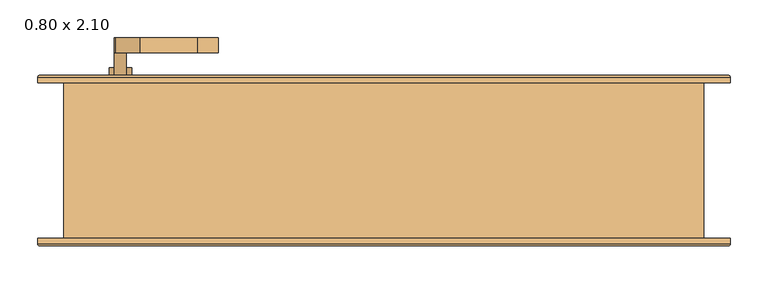
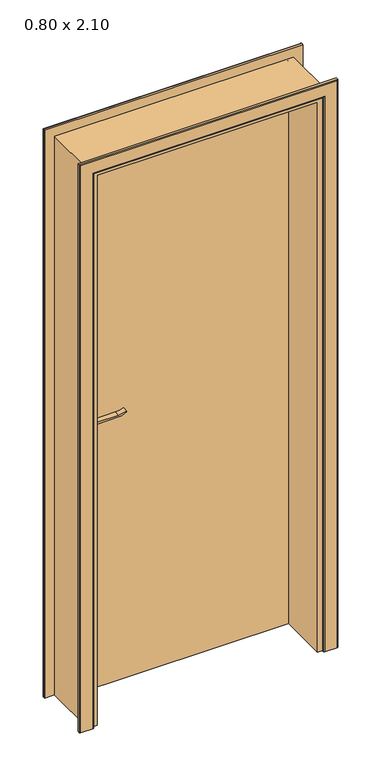
"""IFC4 building model written with IfcOpenShell, lengths in millimetres: door geometry, .CC_ND 300_PORTA SIMPLES DE ABRIR_COM EXTENSÃO : 0.80 x 2.10."""

from ifc_helpers import new_model, si_unit, point, frame, frame_2d, origin, origin_with_axes, place, context, project, spatial, polyline, circle_curve, ellipse_curve, trimmed, segment, composite_curve, outline, extrude, faceted_brep, source, transform, mapped, element, save
from ifc_brep_helpers import plane_surface, cylinder_surface, advanced_brep


def door_0_80_x_2_10_30072744(model_context):
    return source(origin(), model_context, "Body", "SolidModel", [
        extrude(outline(composite_curve([segment(trimmed(circle_curve(frame_2d((964.5, -350.0)), 15.0), [point((964.5, -335.0))], [point((964.5, -365.0))], False, "CARTESIAN"), True, "CONTINUOUS"), segment(trimmed(circle_curve(frame_2d((964.5, -350.0)), 15.0), [point((964.5, -365.0))], [point((964.5, -335.0))], False, "CARTESIAN"), True, "CONTINUOUS")], self_intersect=False)), frame((0.0, 110.7, 0.0), z_axis=(0.0, 1.0, 0.0), x_axis=(0.0, 0.0, 1.0)), (0.0, 0.0, 1.0), 10.0),
        extrude(outline(composite_curve([segment(trimmed(circle_curve(frame_2d((964.5, -350.0)), 15.0), [point((964.5, -335.0))], [point((964.5, -365.0))], False, "CARTESIAN"), True, "CONTINUOUS"), segment(trimmed(circle_curve(frame_2d((964.5, -350.0)), 15.0), [point((964.5, -365.0))], [point((964.5, -335.0))], False, "CARTESIAN"), True, "CONTINUOUS")], self_intersect=False)), frame((0.0, 50.7, 0.0), z_axis=(0.0, 1.0, 0.0), x_axis=(0.0, 0.0, 1.0)), (0.0, 0.0, 1.0), 10.0),
        extrude(outline(composite_curve([segment(trimmed(circle_curve(frame_2d((1024.5, -350.0)), 8.0), [point((1029.1523287, -356.5081363))], [point((1024.5, -342.0))], False, "CARTESIAN"), True, "CONTINUOUS"), segment(trimmed(circle_curve(frame_2d((1019.3738613, -324.6138099)), 18.1261387), [point((1024.5, -342.0))], [point((1037.5, -324.6138099))], True, "CARTESIAN"), True, "CONTINUOUS"), segment(polyline([(1037.5, -324.6138099), (1037.5, -248.3564091)]), True, "CONTINUOUS"), segment(trimmed(circle_curve(frame_2d((1096.7709207, -251.9396612)), 59.3791355), [point((1037.5, -248.3564091))], [point((1046.7135558, -220.0))], False, "CARTESIAN"), True, "CONTINUOUS"), segment(polyline([(1046.7135558, -220.0), (1049.5, -220.0)]), True, "CONTINUOUS"), segment(trimmed(circle_curve(frame_2d((1127.7850638, -248.4227909)), 83.2850902), [point((1049.5, -220.0))], [point((1044.5, -248.3564091))], True, "CARTESIAN"), True, "CONTINUOUS"), segment(polyline([(1044.5, -248.3564091), (1044.5, -324.6325667)]), True, "CONTINUOUS"), segment(trimmed(circle_curve(frame_2d((1007.2555521, -326.3324871)), 37.2832219), [point((1044.5, -324.6325667))], [point((1029.1523287, -356.5081363))], False, "CARTESIAN"), True, "CONTINUOUS")], self_intersect=False)), frame((0.0, 140.7, 0.0), z_axis=(0.0, 1.0, 0.0), x_axis=(0.0, 0.0, 1.0)), (0.0, 0.0, 1.0), 20.0),
        extrude(outline(composite_curve([segment(trimmed(circle_curve(frame_2d((1019.3738682, -324.6138122)), 18.1261318), [point((1024.4999903, -342.0))], [point((1037.5, -324.6138122))], True, "CARTESIAN"), True, "CONTINUOUS"), segment(polyline([(1037.5, -324.6138122), (1037.5, -248.3564091)]), True, "CONTINUOUS"), segment(trimmed(circle_curve(frame_2d((1096.7709207, -251.9396612)), 59.3791355), [point((1037.5, -248.3564091))], [point((1046.7135558, -220.0))], False, "CARTESIAN"), True, "CONTINUOUS"), segment(polyline([(1046.7135558, -220.0), (1049.5, -220.0)]), True, "CONTINUOUS"), segment(trimmed(circle_curve(frame_2d((1127.7850638, -248.4227909)), 83.2850902), [point((1049.5, -220.0))], [point((1044.5, -248.3564091))], True, "CARTESIAN"), True, "CONTINUOUS"), segment(polyline([(1044.5, -248.3564091), (1044.5, -324.6325667)]), True, "CONTINUOUS"), segment(trimmed(circle_curve(frame_2d((1007.2555521, -326.3324871)), 37.2832219), [point((1044.5, -324.6325667))], [point((1029.1523287, -356.5081363))], False, "CARTESIAN"), True, "CONTINUOUS"), segment(trimmed(circle_curve(frame_2d((1024.5, -350.0)), 8.0), [point((1029.1523287, -356.5081363))], [point((1024.4999903, -342.0))], False, "CARTESIAN"), True, "CONTINUOUS")], self_intersect=False)), frame((0.0, 10.7, 0.0), z_axis=(0.0, 1.0, 0.0), x_axis=(0.0, 0.0, 1.0)), (0.0, 0.0, 1.0), 20.0),
        extrude(outline(composite_curve([segment(trimmed(circle_curve(frame_2d((1024.5, -350.0)), 8.0), [point((1024.5, -342.0))], [point((1024.5, -358.0))], False, "CARTESIAN"), True, "CONTINUOUS"), segment(trimmed(circle_curve(frame_2d((1024.5, -350.0)), 8.0), [point((1024.5, -358.0))], [point((1024.5, -342.0))], False, "CARTESIAN"), True, "CONTINUOUS")], self_intersect=False)), frame((0.0, 110.7, 0.0), z_axis=(0.0, 1.0, 0.0), x_axis=(0.0, 0.0, 1.0)), (0.0, 0.0, 1.0), 30.0),
        extrude(outline(composite_curve([segment(trimmed(circle_curve(frame_2d((1024.5, -350.0)), 8.0), [point((1024.5, -342.0))], [point((1024.5, -358.0))], False, "CARTESIAN"), True, "CONTINUOUS"), segment(trimmed(circle_curve(frame_2d((1024.5, -350.0)), 8.0), [point((1024.5, -358.0))], [point((1024.5, -342.0))], False, "CARTESIAN"), True, "CONTINUOUS")], self_intersect=False)), frame((0.0, 30.7, 0.0), z_axis=(0.0, 1.0, 0.0), x_axis=(0.0, 0.0, 1.0)), (0.0, 0.0, 1.0), 30.0),
        extrude(outline(composite_curve([segment(trimmed(circle_curve(frame_2d((954.5, -350.0)), 25.0), [point((954.5, -375.0))], [point((954.5, -325.0))], False, "CARTESIAN"), True, "CONTINUOUS"), segment(polyline([(954.5, -325.0), (1024.5, -325.0)]), True, "CONTINUOUS"), segment(trimmed(circle_curve(frame_2d((1024.5, -350.0)), 25.0), [point((1024.5, -325.0))], [point((1024.5, -375.0))], False, "CARTESIAN"), True, "CONTINUOUS"), segment(polyline([(1024.5, -375.0), (954.5, -375.0)]), True, "CONTINUOUS")], self_intersect=False)), frame((0.0, 100.7, 0.0), z_axis=(0.0, 1.0, 0.0), x_axis=(0.0, 0.0, 1.0)), (0.0, 0.0, 1.0), 10.0),
        extrude(outline(composite_curve([segment(trimmed(circle_curve(frame_2d((954.5, -350.0)), 25.0), [point((954.5, -375.0))], [point((954.5, -325.0))], False, "CARTESIAN"), True, "CONTINUOUS"), segment(polyline([(954.5, -325.0), (1024.5, -325.0)]), True, "CONTINUOUS"), segment(trimmed(circle_curve(frame_2d((1024.5, -350.0)), 25.0), [point((1024.5, -325.0))], [point((1024.5, -375.0))], False, "CARTESIAN"), True, "CONTINUOUS"), segment(polyline([(1024.5, -375.0), (954.5, -375.0)]), True, "CONTINUOUS")], self_intersect=False)), frame((0.0, 60.7, 0.0), z_axis=(0.0, 1.0, 0.0), x_axis=(0.0, 0.0, 1.0)), (0.0, 0.0, 1.0), 10.0),
        faceted_brep([(392.0, -106.0, 0.0), (392.0, 70.7, 0.0), (400.0, 70.7, 0.0), (400.0, 100.7, 0.0), (425.0, 100.7, 0.0), (425.0, -106.0, 0.0), (425.0, -106.0, 2100.0), (-425.0, -106.0, 2100.0), (-425.0, -106.0, 0.0), (-392.0, -106.0, 0.0), (-392.0, -106.0, 2067.0), (392.0, -106.0, 2067.0), (425.0, 100.7, 2100.0), (400.0, 100.7, 2075.0), (-400.0, 100.7, 2075.0), (-400.0, 100.7, 0.0), (-425.0, 100.7, 0.0), (-425.0, 100.7, 2100.0), (400.0, 70.7, 2075.0), (392.0, 70.7, 2067.0), (-392.0, 70.7, 2067.0), (-392.0, 70.7, 0.0), (-400.0, 70.7, 0.0), (-400.0, 70.7, 2075.0)], [[[0, 1, 2, 3, 4, 5]], [[5, 6, 7, 8, 9, 10, 11, 0]], [[4, 12, 6, 5]], [[3, 13, 14, 15, 16, 17, 12, 4]], [[2, 18, 13, 3]], [[1, 19, 20, 21, 22, 23, 18, 2]], [[0, 11, 19, 1]], [[10, 9, 21, 20]], [[9, 8, 16, 15, 22, 21]], [[17, 16, 8, 7]], [[23, 22, 15, 14]], [[12, 17, 7, 6]], [[18, 23, 14, 13]], [[11, 10, 20, 19]]]),
        extrude(outline(polyline([(-400.0, 70.7), (-400.0, 100.7), (400.0, 100.7), (400.0, 70.7), (-400.0, 70.7)])), origin_with_axes(), (0.0, 0.0, 1.0), 2075.0),
        advanced_brep(
        [(-460.0, 100.7, 0.0), (-460.0, 107.7, 0.0), (-457.0, 110.7, 0.0), (-413.0, 110.7, 0.0), (-410.0, 107.7, 0.0), (-410.0, 100.7, 0.0), (-410.0, 100.7, 2085.0), (410.0, 100.7, 2085.0), (410.0, 100.7, 0.0), (460.0, 100.7, 0.0), (460.0, 100.7, 2135.0), (-460.0, 100.7, 2135.0), (-410.0, 107.7, 2085.0), (-413.0, 110.7, 2088.0), (-457.0, 110.7, 2132.0), (457.0, 110.7, 2132.0), (457.0, 110.7, 0.0), (413.0, 110.7, 0.0), (413.0, 110.7, 2088.0), (-460.0, 107.7, 2135.0), (460.0, 107.7, 0.0), (460.0, 107.7, 2135.0), (410.0, 107.7, 0.0), (410.0, 107.7, 2085.0)],
        [
            (0, 1),
            (1, 2, circle_curve(frame((-457.0, 107.7, 0.0), z_axis=(0.0, 0.0, -1.0), x_axis=(1.0, 0.0, 0.0)), 3.0)),
            (2, 3),
            (3, 4, circle_curve(frame((-413.0, 107.7, 0.0), z_axis=(0.0, 0.0, -1.0), x_axis=(1.0, 0.0, 0.0)), 3.0)),
            (4, 5),
            (5, 0),
            (5, 6),
            (6, 7),
            (7, 8),
            (8, 9),
            (9, 10),
            (10, 11),
            (11, 0),
            (4, 12),
            (12, 6),
            (3, 13),
            (13, 12, ellipse_curve(frame((-413.0, 107.7, 2088.0), z_axis=(-0.7071067811865475, 0.0, -0.7071067811865475), x_axis=(0.7071067811865474, 0.0, -0.7071067811865476)), 4.2426407, 3.0)),
            (2, 14),
            (14, 15),
            (15, 16),
            (16, 17),
            (17, 18),
            (18, 13),
            (1, 19),
            (19, 14, ellipse_curve(frame((-457.0, 107.7, 2132.0), z_axis=(-0.7071067811865475, 0.0, -0.7071067811865475), x_axis=(0.7071067811865474, 0.0, -0.7071067811865476)), 4.2426407, 3.0)),
            (11, 19),
            (9, 20),
            (20, 21),
            (21, 10),
            (8, 22),
            (22, 17, circle_curve(frame((413.0, 107.7, 0.0), z_axis=(0.0, 0.0, -1.0), x_axis=(-1.0, 0.0, 0.0)), 3.0)),
            (16, 20, circle_curve(frame((457.0, 107.7, 0.0), z_axis=(0.0, 0.0, -1.0), x_axis=(-1.0, 0.0, 0.0)), 3.0)),
            (23, 22),
            (7, 23),
            (23, 18, ellipse_curve(frame((413.0, 107.7, 2088.0), z_axis=(0.7071067811865475, 0.0, -0.7071067811865475), x_axis=(0.7071067811865474, 0.0, 0.7071067811865476)), 4.2426407, 3.0)),
            (15, 21, ellipse_curve(frame((457.0, 107.7, 2132.0), z_axis=(0.7071067811865475, 0.0, -0.7071067811865475), x_axis=(0.7071067811865474, 0.0, 0.7071067811865476)), 4.2426407, 3.0)),
            (12, 23),
            (21, 19),
        ],
        [
            plane_surface(frame((-410.0, 100.7, 0.0), z_axis=(0.0, 0.0, -1.0), x_axis=(0.0, -1.0, 0.0))),
            plane_surface(frame((-460.0, 100.7, 0.0), z_axis=(0.0, -1.0, 0.0), x_axis=(0.0, 0.0, 1.0))),
            plane_surface(frame((-410.0, 100.7, 0.0), z_axis=(1.0, 0.0, 0.0), x_axis=(0.0, 0.0, 1.0))),
            cylinder_surface(frame((-413.0, 107.7, 0.0), z_axis=(0.0, 0.0, -1.0), x_axis=(1.0, 0.0, 0.0)), 3.0),
            plane_surface(frame((-413.0, 110.7, 0.0), z_axis=(0.0, 1.0, 0.0), x_axis=(0.0, 0.0, 1.0))),
            cylinder_surface(frame((-457.0, 107.7, 0.0), z_axis=(0.0, 0.0, -1.0), x_axis=(1.0, 0.0, 0.0)), 3.0),
            plane_surface(frame((-460.0, 107.7, 0.0), z_axis=(-1.0, 0.0, 0.0), x_axis=(0.0, 0.0, 1.0))),
            plane_surface(frame((460.0, 107.7, 2135.0), z_axis=(1.0, 0.0, 0.0), x_axis=(0.0, 0.0, -1.0))),
            plane_surface(frame((410.0, 100.7, 0.0), z_axis=(0.0, 0.0, -1.0), x_axis=(0.0, -1.0, 0.0))),
            plane_surface(frame((410.0, 100.7, 2085.0), z_axis=(-1.0, 0.0, 0.0), x_axis=(0.0, 0.0, -1.0))),
            cylinder_surface(frame((413.0, 107.7, 2085.0), z_axis=(0.0, 0.0, 1.0), x_axis=(-1.0, 0.0, 0.0)), 3.0),
            cylinder_surface(frame((457.0, 107.7, 2085.0), z_axis=(0.0, 0.0, 1.0), x_axis=(-1.0, 0.0, 0.0)), 3.0),
            plane_surface(frame((-410.0, 100.7, 2085.0), z_axis=(0.0, 0.0, -1.0), x_axis=(1.0, 0.0, 0.0))),
            plane_surface(frame((-460.0, 107.7, 2135.0), z_axis=(0.0, 0.0, 1.0), x_axis=(1.0, 0.0, 0.0))),
            cylinder_surface(frame((-410.0, 107.7, 2088.0), z_axis=(-1.0, 0.0, 0.0), x_axis=(0.0, 0.0, -1.0)), 3.0),
            cylinder_surface(frame((-410.0, 107.7, 2132.0), z_axis=(-1.0, 0.0, 0.0), x_axis=(0.0, 0.0, -1.0)), 3.0),
        ],
        [
            (0, [[1, 2, 3, 4, 5, 6]]),
            (1, [[7, 8, 9, 10, 11, 12, 13, -6]]),
            (2, [[14, 15, -7, -5]]),
            (3, [[16, 17, -14, -4]]),
            (4, [[18, 19, 20, 21, 22, 23, -16, -3]]),
            (5, [[24, 25, -18, -2]]),
            (6, [[-13, 26, -24, -1]]),
            (7, [[-11, 27, 28, 29]]),
            (8, [[-10, 30, 31, -21, 32, -27]]),
            (9, [[33, -30, -9, 34]]),
            (10, [[-22, -31, -33, 35]]),
            (11, [[-28, -32, -20, 36]]),
            (12, [[37, -34, -8, -15]]),
            (13, [[-12, -29, 38, -26]]),
            (14, [[-23, -35, -37, -17]]),
            (15, [[-38, -36, -19, -25]]),
        ],
    ),
        advanced_brep(
        [(460.0, -106.0, 0.0), (460.0, -113.0342217, 0.0), (457.0342217, -116.0, 0.0), (412.9842717, -116.0, 0.0), (410.0, -113.0157283, 0.0), (410.0, -106.0, 0.0), (410.0, -106.0, 2085.0), (-410.0, -106.0, 2085.0), (-410.0, -106.0, 0.0), (-460.0, -106.0, 0.0), (-460.0, -106.0, 2135.0), (460.0, -106.0, 2135.0), (410.0, -113.0157283, 2085.0), (412.9842717, -116.0, 2087.9842717), (457.0342217, -116.0, 2132.0342217), (-457.0342217, -116.0, 2132.0342217), (-457.0342217, -116.0, 0.0), (-412.9842717, -116.0, 0.0), (-412.9842717, -116.0, 2087.9842717), (460.0, -113.0342217, 2135.0), (-460.0, -113.0342217, 0.0), (-460.0, -113.0342217, 2135.0), (-410.0, -113.0157283, 0.0), (-410.0, -113.0157283, 2085.0)],
        [
            (0, 1),
            (1, 2, circle_curve(frame((457.0342217, -113.0342217, 0.0), z_axis=(0.0, 0.0, -1.0), x_axis=(1.0, 0.0, 0.0)), 2.9657783)),
            (2, 3),
            (3, 4, circle_curve(frame((412.9842717, -113.0157283, 0.0), z_axis=(0.0, 0.0, -1.0), x_axis=(1.0, 0.0, 0.0)), 2.9842717)),
            (4, 5),
            (5, 0),
            (5, 6),
            (6, 7),
            (7, 8),
            (8, 9),
            (9, 10),
            (10, 11),
            (11, 0),
            (4, 12),
            (12, 6),
            (3, 13),
            (13, 12, ellipse_curve(frame((412.9842717, -113.0157283, 2087.9842717), z_axis=(0.7071067811865475, 0.0, -0.7071067811865475), x_axis=(-0.7071067811865474, 0.0, -0.7071067811865476)), 4.2203975, 2.9842717)),
            (2, 14),
            (14, 15),
            (15, 16),
            (16, 17),
            (17, 18),
            (18, 13),
            (1, 19),
            (19, 14, ellipse_curve(frame((457.0342217, -113.0342217, 2132.0342217), z_axis=(0.7071067811865475, 0.0, -0.7071067811865475), x_axis=(-0.7071067811865474, 0.0, -0.7071067811865476)), 4.1942438, 2.9657783)),
            (11, 19),
            (9, 20),
            (20, 21),
            (21, 10),
            (8, 22),
            (22, 17, circle_curve(frame((-412.9842717, -113.0157283, 0.0), z_axis=(0.0, 0.0, -1.0), x_axis=(-1.0, 0.0, 0.0)), 2.9842717)),
            (16, 20, circle_curve(frame((-457.0342217, -113.0342217, 0.0), z_axis=(0.0, 0.0, -1.0), x_axis=(-1.0, 0.0, 0.0)), 2.9657783)),
            (23, 22),
            (7, 23),
            (23, 18, ellipse_curve(frame((-412.9842717, -113.0157283, 2087.9842717), z_axis=(-0.7071067811865475, 0.0, -0.7071067811865475), x_axis=(-0.7071067811865474, 0.0, 0.7071067811865476)), 4.2203975, 2.9842717)),
            (15, 21, ellipse_curve(frame((-457.0342217, -113.0342217, 2132.0342217), z_axis=(-0.7071067811865475, 0.0, -0.7071067811865475), x_axis=(-0.7071067811865474, 0.0, 0.7071067811865476)), 4.1942438, 2.9657783)),
            (12, 23),
            (21, 19),
        ],
        [
            plane_surface(frame((410.0, -106.0, 0.0), z_axis=(0.0, 0.0, -1.0), x_axis=(0.0, -1.0, 0.0))),
            plane_surface(frame((460.0, -106.0, 0.0), z_axis=(0.0, 1.0, 0.0), x_axis=(0.0, 0.0, 1.0))),
            plane_surface(frame((410.0, -106.0, 0.0), z_axis=(-1.0, 0.0, 0.0), x_axis=(0.0, 0.0, 1.0))),
            cylinder_surface(frame((412.9842717, -113.0157283, 0.0), z_axis=(0.0, 0.0, -1.0), x_axis=(1.0, 0.0, 0.0)), 2.9842717),
            plane_surface(frame((412.9842717, -116.0, 0.0), z_axis=(0.0, -1.0, 0.0), x_axis=(0.0, 0.0, 1.0))),
            cylinder_surface(frame((457.0342217, -113.0342217, 0.0), z_axis=(0.0, 0.0, -1.0), x_axis=(1.0, 0.0, 0.0)), 2.9657783),
            plane_surface(frame((460.0, -113.0342217, 0.0), z_axis=(1.0, 0.0, 0.0), x_axis=(0.0, 0.0, 1.0))),
            plane_surface(frame((-460.0, -113.0342217, 2135.0), z_axis=(-1.0, 0.0, 0.0), x_axis=(0.0, 0.0, -1.0))),
            plane_surface(frame((-410.0, -106.0, 0.0), z_axis=(0.0, 0.0, -1.0), x_axis=(0.0, -1.0, 0.0))),
            plane_surface(frame((-410.0, -106.0, 2085.0), z_axis=(1.0, 0.0, 0.0), x_axis=(0.0, 0.0, -1.0))),
            cylinder_surface(frame((-412.9842717, -113.0157283, 2085.0), z_axis=(0.0, 0.0, 1.0), x_axis=(-1.0, 0.0, 0.0)), 2.9842717),
            cylinder_surface(frame((-457.0342217, -113.0342217, 2085.0), z_axis=(0.0, 0.0, 1.0), x_axis=(-1.0, 0.0, 0.0)), 2.9657783),
            plane_surface(frame((410.0, -106.0, 2085.0), z_axis=(0.0, 0.0, -1.0), x_axis=(-1.0, 0.0, 0.0))),
            plane_surface(frame((460.0, -113.0342217, 2135.0), z_axis=(0.0, 0.0, 1.0), x_axis=(-1.0, 0.0, 0.0))),
            cylinder_surface(frame((410.0, -113.0157283, 2087.9842717), z_axis=(1.0, 0.0, 0.0), x_axis=(0.0, 0.0, 1.0)), 2.9842717),
            cylinder_surface(frame((410.0, -113.0342217, 2132.0342217), z_axis=(1.0, 0.0, 0.0), x_axis=(0.0, 0.0, 1.0)), 2.9657783),
        ],
        [
            (0, [[1, 2, 3, 4, 5, 6]]),
            (1, [[7, 8, 9, 10, 11, 12, 13, -6]]),
            (2, [[14, 15, -7, -5]]),
            (3, [[16, 17, -14, -4]]),
            (4, [[18, 19, 20, 21, 22, 23, -16, -3]]),
            (5, [[24, 25, -18, -2]]),
            (6, [[-13, 26, -24, -1]]),
            (7, [[-11, 27, 28, 29]]),
            (8, [[-10, 30, 31, -21, 32, -27]]),
            (9, [[33, -30, -9, 34]]),
            (10, [[-22, -31, -33, 35]]),
            (11, [[-28, -32, -20, 36]]),
            (12, [[37, -34, -8, -15]]),
            (13, [[-12, -29, 38, -26]]),
            (14, [[-23, -35, -37, -17]]),
            (15, [[-38, -36, -19, -25]]),
        ],
    ),
    ])


if __name__ == "__main__":
    model = new_model("IFC4")
    model_context = context("Model", 3, world=origin())
    ifc_project = project(units=[si_unit("LENGTHUNIT", "METRE", prefix="MILLI")], contexts=[model_context])
    site = spatial("IfcSite", under=ifc_project)
    building = spatial("IfcBuilding", under=site)
    placement = place(None, origin())
    door_0_80_x_2_10_shape = door_0_80_x_2_10_30072744(model_context)
    element("IfcDoor", 1, ObjectType=".CC_ND 300_PORTA SIMPLES DE ABRIR_COM EXTENSÃO : 0.80 x 2.10", at=placement, inside=building, context=model_context, shape_type="MappedRepresentation", body=[
        mapped(door_0_80_x_2_10_shape, transform((0.0, 0.0, 0.0), x_axis=(1.0, 0.0, 0.0), y_axis=(0.0, 1.0, 0.0), z_axis=(0.0, 0.0, 1.0))),
    ])
    save(model, "model.ifc")

# Revit data of these elements
# Type ".CC_ND 300_PORTA SIMPLES DE ABRIR_COM EXTENSÃO : 0.80 x 2.10"
#   Type Mark = "153"
#   Analytic Construction = "<None>"
#   Rough Width = 0.85 m
#   Espessura moldura externa = 0.01 m
#   Espessura moldura interna = 0.01 m
#   Largura moldura = 0.05 m
#   Extensão acabamento exterior [instance default] = 0.00 m
#   Extensão acabamento interior [instance default] = 0.00 m
#   Espessura batente = 0.025 m
#   Thickness = 0.03 m
#   Altura batente = 2.085 m
#   Aux Arco [instance default] = 0.80 m
#   Rough Height = 2.125 m
#   Height = 2.10 m
#   Width = 0.80 m
#   Moldura interna [instance default] = yes
#   Moldura externa [instance default] = yes
#   Porta = .MADEIRA COM PINTURA ESMALTE BRANCO ACETINADO
#   Moldura = .MADEIRA COM PINTURA ESMALTE BRANCO ACETINADO
#   Maçaneta = .ALUMÍNIO
#   Batente = .MADEIRA COM PINTURA ESMALTE BRANCO ACETINADO
#   Function = (empty or 0)
#   Wall Closure = (empty or 0)
# Element 1 (IfcDoor, ".CC_ND 300_PORTA SIMPLES DE ABRIR_COM EXTENSÃO : 0.80 x 2.10")
#   Extensão acabamento exterior = 0.031 m
#   Extensão acabamento interior = 0.0257 m
#   Aux Arco = 0.8257 m
#   Materials on its faces: ".MADEIRA COM PINTURA ESMALTE BRANCO ACETINADO", ".ALUMÍNIO"
# Materials
#   ".MADEIRA COM PINTURA ESMALTE BRANCO ACETINADO": class ".CC_MADEIRAS", colour RGB 240 240 240, transparency 0, Description = "Madeira com pintura esmalte branco acetinado.", Cost = 0
#   ".ALUMÍNIO": class "CC_METAIS", colour RGB 244 244 244, transparency 0, Description = "Material alumínio", Cost = 0
